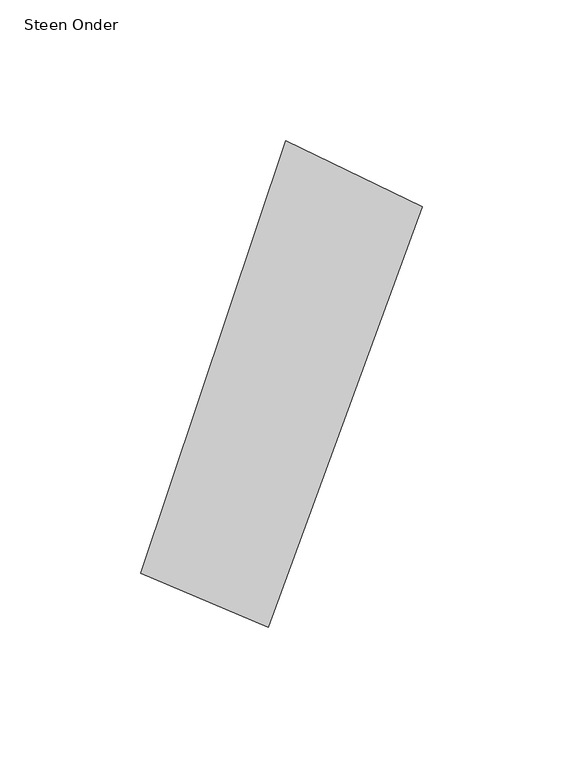
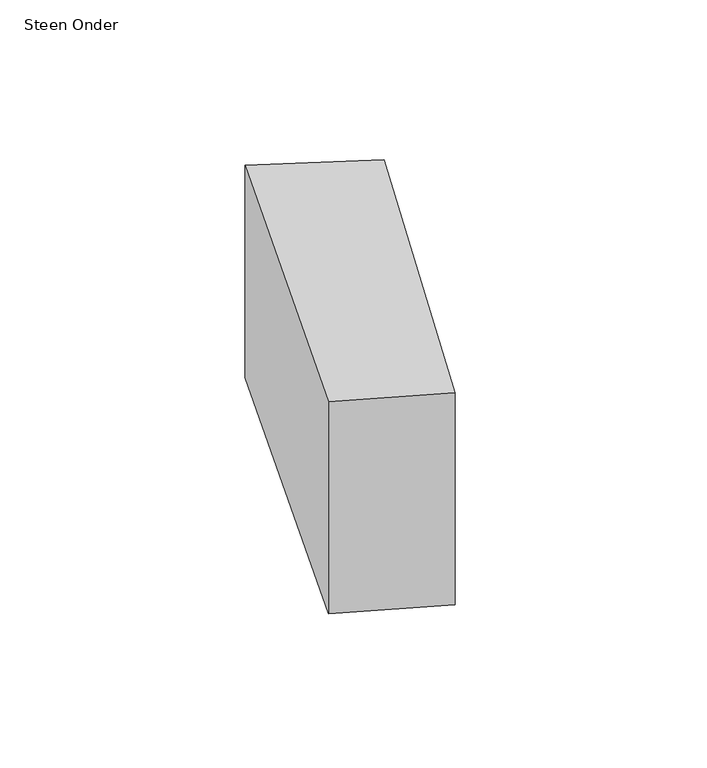
"""IFC4 building model written with IfcOpenShell, lengths in millimetres: proxy geometry, 00_GMA_steen_versie_4 : Steen Onder."""

from ifc_helpers import new_model, si_unit, origin, origin_with_axes, place, context, project, spatial, polyline, outline, extrude, source, transform, mapped, element, save


def steen_onder_8dfde7b8(model_context):
    return source(origin(), model_context, "Body", "SweptSolid", [
        extrude(outline(polyline([(127.5293573, 143.142917), (72.857299, -6.2802458), (27.4472893, 12.8985949), (79.0710287, 166.6705794), (127.5293573, 143.142917)])), origin_with_axes(), (0.0, 0.0, 1.0), 100.0),
    ])


if __name__ == "__main__":
    model = new_model("IFC4")
    model_context = context("Model", 3, world=origin())
    ifc_project = project(units=[si_unit("LENGTHUNIT", "METRE", prefix="MILLI")], contexts=[model_context])
    site = spatial("IfcSite", under=ifc_project)
    building = spatial("IfcBuilding", under=site)
    placement = place(None, origin())
    steen_onder_shape = steen_onder_8dfde7b8(model_context)
    element("IfcBuildingElementProxy", 1, Name="00_GMA_steen_versie_4 : Steen Onder", ObjectType="00_GMA_steen_versie_4 : Steen Onder", at=placement, inside=building, context=model_context, shape_type="MappedRepresentation", body=[
        mapped(steen_onder_shape, transform((0.0, 0.0, 0.0), x_axis=(1.0, 0.0, 0.0), y_axis=(0.0, 1.0, 0.0), z_axis=(0.0, 0.0, 1.0))),
    ])
    save(model, "model.ifc")

# Revit data of these elements
# Type "00_GMA_steen_versie_4 : Steen Onder"
#   StootVoegHalfBoven [instance default] = 5 mm
#   StootVoegHalf [instance default] = 5 mm
#   StootVoegBreedteOnder = 10 mm
#   StootVoegBreedteBoven = 10 mm
#   Steendikte = 100 mm
#   LintVoegOnderHalf = 0 mm
#   LintVoegOnder = 0 mm
#   LintVoegBovenHalf = 5 mm
#   LintVoegBoven = 10 mm
#   materiaal = none
#   MateriaalVoeg = none
#   Default Elevation = 0
